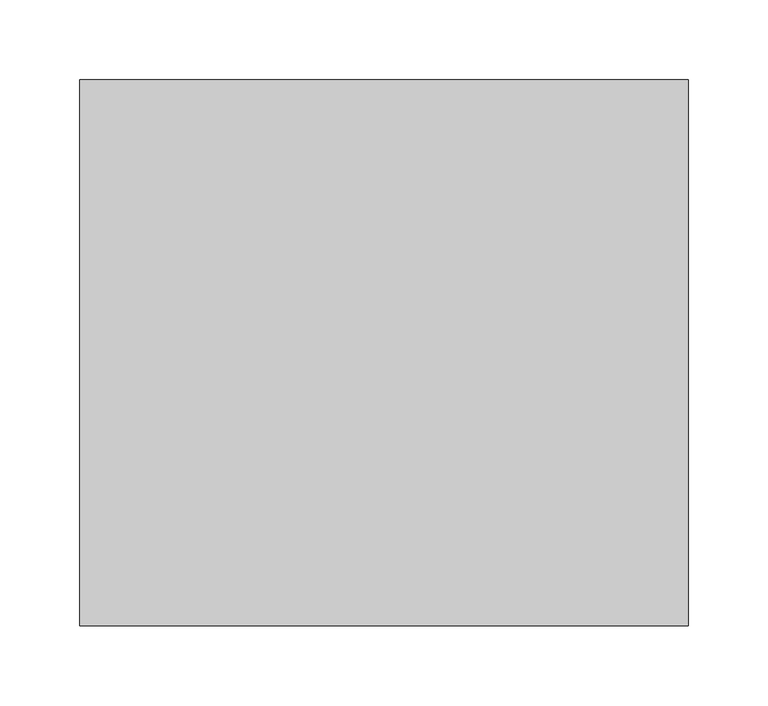
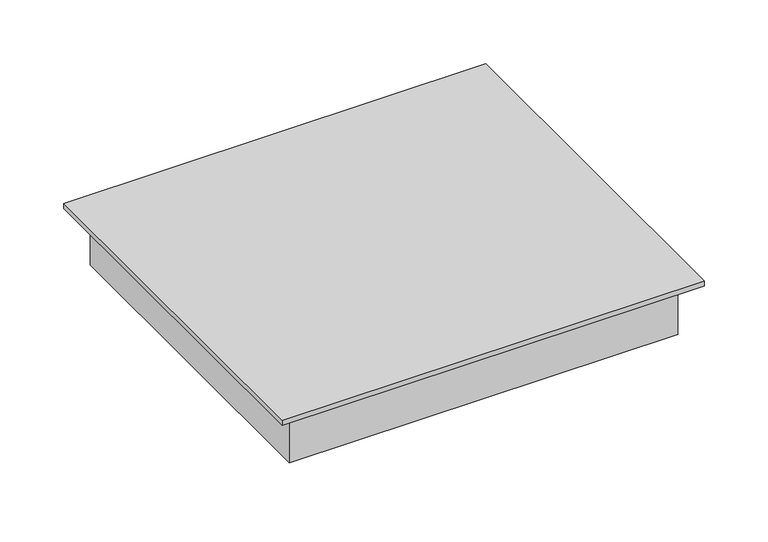
"""IFC4 building model written with IfcOpenShell, lengths in millimetres: proxy geometry, CAIXA VERTICE V7 : QD Amanco Passagem Grande."""

from ifc_helpers import new_model, si_unit, origin, origin_with_axes, place, context, project, spatial, polyline, outline, extrude, faceted_brep, source, transform, mapped, element, save


def electrical_fixtures_5770d9fd(model_context):
    return source(origin(), model_context, "Body", "SolidModel", [
        faceted_brep([(173.5, 946.0, -48.0), (173.5, 1254.0, -48.0), (-173.5, 1254.0, -48.0), (-173.5, 946.0, -48.0), (175.5, 1256.0, -50.0), (175.5, 944.0, -50.0), (-175.5, 944.0, -50.0), (-175.5, 1256.0, -50.0), (-175.5, 1256.0, 0.0), (175.5, 1256.0, 0.0), (-175.5, 944.0, 0.0), (175.5, 944.0, 0.0), (173.5, 1254.0, 0.0), (173.5, 946.0, 0.0), (-173.5, 946.0, 0.0), (-173.5, 1254.0, 0.0)], [[[0, 1, 2, 3]], [[4, 5, 6, 7]], [[4, 7, 8, 9]], [[8, 7, 6, 10]], [[10, 6, 5, 11]], [[11, 5, 4, 9]], [[9, 8, 10, 11], [12, 13, 14, 15]], [[13, 12, 1, 0]], [[14, 13, 0, 3]], [[15, 14, 3, 2]], [[12, 15, 2, 1]]]),
        extrude(outline(polyline([(190.5, 1271.0), (190.5, 929.0), (-190.5, 929.0), (-190.5, 1271.0), (190.5, 1271.0)])), origin_with_axes(), (0.0, 0.0, 1.0), 5.0),
    ])


if __name__ == "__main__":
    model = new_model("IFC4")
    model_context = context("Model", 3, world=origin())
    ifc_project = project(units=[si_unit("LENGTHUNIT", "METRE", prefix="MILLI")], contexts=[model_context])
    site = spatial("IfcSite", under=ifc_project)
    building = spatial("IfcBuilding", under=site)
    placement = place(None, origin())
    electrical_fixtures_shape = electrical_fixtures_5770d9fd(model_context)
    element("IfcBuildingElementProxy", 1, Name="CAIXA VERTICE V7 : QD Amanco Passagem Grande", ObjectType="CAIXA VERTICE V7 : QD Amanco Passagem Grande", at=placement, inside=building, context=model_context, shape_type="MappedRepresentation", body=[
        mapped(electrical_fixtures_shape, transform((0.0, 0.0, 0.0), x_axis=(1.0, 0.0, 0.0), y_axis=(0.0, 1.0, 0.0), z_axis=(0.0, 0.0, 1.0))),
    ])
    save(model, "model.ifc")

# Revit data of these elements
# Type "CAIXA VERTICE V7 : QD Amanco Passagem Grande"
#   URL = "www.facebook.com/verticetreinamentos"
#   SEÇÃO [instance default] = ""
#   Rotação [instance default] = 0.00°
#   LARGURA DA TAMPA = 0.381 m
#   BORDA = 0.03 m
#   ALTURA DE INSTALAÇÃO [instance default] = 1.10 m
#   Distância Anotação [instance default] = 0.0015 m
#   ALTURA DA TAMPA = 0.342 m
#   Vertical [instance default] = yes
#   VER SEÇÃO [instance default] = no
#   SHADE ESQ [instance default] = no
#   SHADE DIR [instance default] = yes
#   HORIZONTAL [instance default] = no
#   ANDAR COM A LEGENDA [instance default] = 0
#   Material Tampa [instance default] = Plástico, branco opaco
#   Caixa = element 1798542
#   Anotação = element 1798539
#   Default Elevation = 0
# Element 1 (IfcBuildingElementProxy, "CAIXA VERTICE V7 : QD Amanco Passagem Grande")
#   Materials on its faces: "Plástico, branco opaco"
# Materials
#   "Plástico, branco opaco": class "Plástico", colour RGB 120 120 120, transparency 0, Description = "Plastic, generic, opaque white", Cost = 0
